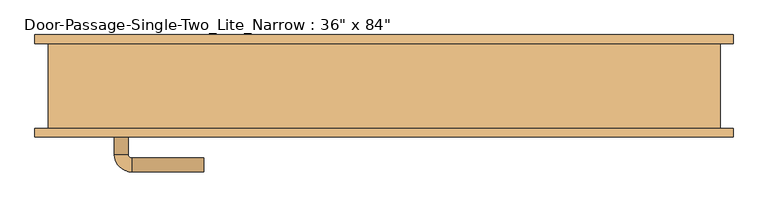
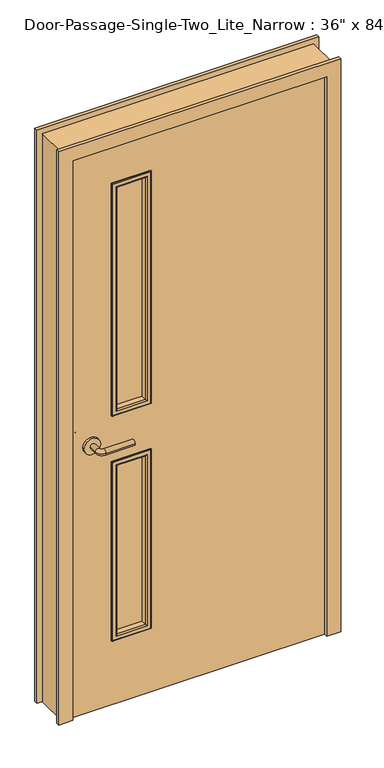
"""IFC4 building model written with IfcOpenShell, lengths in millimetres: door geometry."""

from ifc_helpers import new_model, si_unit, point, frame, frame_2d, origin, place, context, project, spatial, polyline, circle_curve, ellipse_curve, trimmed, segment, composite_curve, outline, extrude, faceted_brep, source, transform, mapped, element, save
from ifc_brep_helpers import plane_surface, cylinder_surface, revolved_surface, advanced_brep


def door_7eef6684(model_context):
    return source(origin(), model_context, "Body", "SolidModel", [
        advanced_brep(
        [(-392.190625, -15.8125, 1016.0), (-372.190625, -15.8125, 1016.0), (-392.190625, 14.1875, 1016.0), (-372.190625, 14.1875, 1016.0), (-367.190625, 19.1875, 1016.0), (-367.190625, 39.1875, 1016.0), (-262.190625, 39.1875, 1016.0), (-262.190625, 19.1875, 1016.0)],
        [
            (0, 1, circle_curve(frame((-382.190625, -15.8125, 1016.0), z_axis=(0.0, -1.0, 0.0), x_axis=(1.0, 0.0, 0.0)), 10.0)),
            (1, 0, circle_curve(frame((-382.190625, -15.8125, 1016.0), z_axis=(0.0, -1.0, 0.0), x_axis=(1.0, 0.0, 0.0)), 10.0)),
            (0, 2),
            (2, 3, circle_curve(frame((-382.190625, 14.1875, 1016.0), z_axis=(0.0, -1.0, 0.0), x_axis=(1.0, 0.0, 0.0)), 10.0)),
            (3, 1),
            (3, 2, circle_curve(frame((-382.190625, 14.1875, 1016.0), z_axis=(0.0, -1.0, 0.0), x_axis=(1.0, 0.0, 0.0)), 10.0)),
            (4, 3, circle_curve(frame((-367.190625, 14.1875, 1016.0), z_axis=(0.0, 0.0, 1.0), x_axis=(-1.0, 0.0, 0.0)), 5.0)),
            (2, 5, circle_curve(frame((-367.190625, 14.1875, 1016.0), z_axis=(0.0, 0.0, -1.0), x_axis=(-1.0, 0.0, 0.0)), 25.0)),
            (5, 4, circle_curve(frame((-367.190625, 29.1875, 1016.0), z_axis=(-1.0, 0.0, 0.0), x_axis=(0.0, -1.0, 0.0)), 10.0)),
            (4, 5, circle_curve(frame((-367.190625, 29.1875, 1016.0), z_axis=(-1.0, 0.0, 0.0), x_axis=(0.0, -1.0, 0.0)), 10.0)),
            (6, 7, circle_curve(frame((-262.190625, 29.1875, 1016.0), z_axis=(1.0, 0.0, 0.0), x_axis=(0.0, -1.0, 0.0)), 10.0)),
            (7, 6, circle_curve(frame((-262.190625, 29.1875, 1016.0), z_axis=(1.0, 0.0, 0.0), x_axis=(0.0, -1.0, 0.0)), 10.0)),
            (5, 6),
            (7, 4),
        ],
        [
            plane_surface(frame((-382.190625, -15.8125, 1016.0), z_axis=(0.0, -1.0, 0.0), x_axis=(0.0, 0.0, 1.0))),
            cylinder_surface(frame((-382.190625, -15.8125, 1016.0), z_axis=(0.0, -1.0, 0.0), x_axis=(1.0, 0.0, 0.0)), 10.0),
            revolved_surface(trimmed(ellipse_curve(frame((-382.190625, 14.1875, 1016.0), z_axis=(0.0, -1.0, 0.0), x_axis=(1.0, 0.0, 0.0)), 10.0, 10.0), [point((-392.190625, 14.1875, 1016.0))], [point((-372.190625, 14.1875, 1016.0))], True, "CARTESIAN"), (-367.190625, 14.1875, 1016.0), (0.0, 0.0, -1.0)),
            revolved_surface(trimmed(ellipse_curve(frame((-382.190625, 14.1875, 1016.0), z_axis=(0.0, -1.0, 0.0), x_axis=(1.0, 0.0, 0.0)), 10.0, 10.0), [point((-372.190625, 14.1875, 1016.0))], [point((-392.190625, 14.1875, 1016.0))], True, "CARTESIAN"), (-367.190625, 14.1875, 1016.0), (0.0, 0.0, -1.0)),
            plane_surface(frame((-262.190625, 29.1875, 1016.0), z_axis=(1.0, 0.0, 0.0), x_axis=(0.0, 0.0, 1.0))),
            cylinder_surface(frame((-367.190625, 29.1875, 1016.0), z_axis=(-1.0, 0.0, 0.0), x_axis=(0.0, -1.0, 0.0)), 10.0),
        ],
        [
            (0, [[1, 2]]),
            (1, [[-1, 3, 4, 5]]),
            (1, [[-2, -5, 6, -3]]),
            (2, [[7, -4, 8, 9]]),
            (3, [[-8, -6, -7, 10]]),
            (4, [[11, 12]]),
            (5, [[-9, 13, -12, 14]]),
            (5, [[-10, -14, -11, -13]]),
        ],
    ),
        extrude(outline(composite_curve([segment(trimmed(circle_curve(frame_2d((1016.0, -384.690625)), 30.0), [point((1016.0, -414.690625))], [point((1016.0, -354.690625))], False, "CARTESIAN"), True, "CONTINUOUS"), segment(trimmed(circle_curve(frame_2d((1016.0, -384.690625)), 30.0), [point((1016.0, -354.690625))], [point((1016.0, -414.690625))], False, "CARTESIAN"), True, "CONTINUOUS")], self_intersect=False)), frame((0.0, -23.8125, 0.0), z_axis=(0.0, 1.0, 0.0), x_axis=(0.0, 0.0, 1.0)), (0.0, 0.0, 1.0), 8.0),
        advanced_brep(
        [(-392.190625, -76.2625, 1016.0), (-372.190625, -76.2625, 1016.0), (-372.190625, -106.2625, 1016.0), (-392.190625, -106.2625, 1016.0), (-367.190625, -111.2625, 1016.0), (-367.190625, -131.2625, 1016.0), (-262.190625, -131.2625, 1016.0), (-262.190625, -111.2625, 1016.0)],
        [
            (0, 1, circle_curve(frame((-382.190625, -76.2625, 1016.0), z_axis=(0.0, 1.0, 0.0), x_axis=(1.0, 0.0, 0.0)), 10.0)),
            (1, 0, circle_curve(frame((-382.190625, -76.2625, 1016.0), z_axis=(0.0, 1.0, 0.0), x_axis=(1.0, 0.0, 0.0)), 10.0)),
            (1, 2),
            (2, 3, circle_curve(frame((-382.190625, -106.2625, 1016.0), z_axis=(0.0, 1.0, 0.0), x_axis=(1.0, 0.0, 0.0)), 10.0)),
            (3, 0),
            (3, 2, circle_curve(frame((-382.190625, -106.2625, 1016.0), z_axis=(0.0, 1.0, 0.0), x_axis=(1.0, 0.0, 0.0)), 10.0)),
            (4, 5, circle_curve(frame((-367.190625, -121.2625, 1016.0), z_axis=(-1.0, 0.0, 0.0), x_axis=(0.0, 1.0, 0.0)), 10.0)),
            (5, 3, circle_curve(frame((-367.190625, -106.2625, 1016.0), z_axis=(0.0, 0.0, -1.0), x_axis=(-1.0, 0.0, 0.0)), 25.0)),
            (2, 4, circle_curve(frame((-367.190625, -106.2625, 1016.0), z_axis=(0.0, 0.0, 1.0), x_axis=(-1.0, 0.0, 0.0)), 5.0)),
            (5, 4, circle_curve(frame((-367.190625, -121.2625, 1016.0), z_axis=(-1.0, 0.0, 0.0), x_axis=(0.0, 1.0, 0.0)), 10.0)),
            (6, 7, circle_curve(frame((-262.190625, -121.2625, 1016.0), z_axis=(1.0, 0.0, 0.0), x_axis=(0.0, 1.0, 0.0)), 10.0)),
            (7, 6, circle_curve(frame((-262.190625, -121.2625, 1016.0), z_axis=(1.0, 0.0, 0.0), x_axis=(0.0, 1.0, 0.0)), 10.0)),
            (4, 7),
            (6, 5),
        ],
        [
            plane_surface(frame((-382.190625, -76.2625, 1016.0), z_axis=(0.0, 1.0, 0.0), x_axis=(0.0, 0.0, 1.0))),
            cylinder_surface(frame((-382.190625, -76.2625, 1016.0), z_axis=(0.0, 1.0, 0.0), x_axis=(1.0, 0.0, 0.0)), 10.0),
            revolved_surface(trimmed(ellipse_curve(frame((-382.190625, -106.2625, 1016.0), z_axis=(0.0, -1.0, 0.0), x_axis=(1.0, 0.0, 0.0)), 10.0, 10.0), [point((-392.190625, -106.2625, 1016.0))], [point((-372.190625, -106.2625, 1016.0))], True, "CARTESIAN"), (-367.190625, -106.2625, 1016.0), (0.0, 0.0, -1.0)),
            revolved_surface(trimmed(ellipse_curve(frame((-382.190625, -106.2625, 1016.0), z_axis=(0.0, -1.0, 0.0), x_axis=(1.0, 0.0, 0.0)), 10.0, 10.0), [point((-372.190625, -106.2625, 1016.0))], [point((-392.190625, -106.2625, 1016.0))], True, "CARTESIAN"), (-367.190625, -106.2625, 1016.0), (0.0, 0.0, -1.0)),
            plane_surface(frame((-262.190625, -121.2625, 1016.0), z_axis=(1.0, 0.0, 0.0), x_axis=(0.0, 0.0, 1.0))),
            cylinder_surface(frame((-367.190625, -121.2625, 1016.0), z_axis=(-1.0, 0.0, 0.0), x_axis=(0.0, 1.0, 0.0)), 10.0),
        ],
        [
            (0, [[1, 2]]),
            (1, [[3, 4, 5, -2]]),
            (1, [[-5, 6, -3, -1]]),
            (2, [[7, 8, -4, 9]]),
            (3, [[10, -9, -6, -8]]),
            (4, [[11, 12]]),
            (5, [[13, -11, 14, -7]]),
            (5, [[-14, -12, -13, -10]]),
        ],
    ),
        extrude(outline(composite_curve([segment(trimmed(circle_curve(frame_2d((1016.0, -384.690625)), 30.0), [point((1016.0, -414.690625))], [point((1016.0, -354.690625))], False, "CARTESIAN"), True, "CONTINUOUS"), segment(trimmed(circle_curve(frame_2d((1016.0, -384.690625)), 30.0), [point((1016.0, -354.690625))], [point((1016.0, -414.690625))], False, "CARTESIAN"), True, "CONTINUOUS")], self_intersect=False)), frame((0.0, -76.2625, 0.0), z_axis=(0.0, 1.0, 0.0), x_axis=(0.0, 0.0, 1.0)), (0.0, 0.0, 1.0), 8.0),
        faceted_brep([(457.2, -80.9625, 0.0), (457.2, -19.05, 0.0), (441.325, -19.05, 0.0), (441.325, 19.05, 0.0), (457.2, 19.05, 0.0), (457.2, 68.2625, 0.0), (508.0, 68.2625, 0.0), (508.0, 55.5625, 0.0), (488.95, 55.5625, 0.0), (488.95, -68.2625, 0.0), (508.0, -68.2625, 0.0), (508.0, -80.9625, 0.0), (508.0, -80.9625, 2184.4), (-508.0, -80.9625, 2184.4), (-508.0, -80.9625, 0.0), (-457.2, -80.9625, 0.0), (-457.2, -80.9625, 2133.6), (457.2, -80.9625, 2133.6), (508.0, -68.2625, 2184.4), (488.95, -68.2625, 2165.35), (-488.95, -68.2625, 2165.35), (-488.95, -68.2625, 0.0), (-508.0, -68.2625, 0.0), (-508.0, -68.2625, 2184.4), (488.95, 55.5625, 2165.35), (508.0, 55.5625, 2184.4), (-508.0, 55.5625, 2184.4), (-508.0, 55.5625, 0.0), (-488.95, 55.5625, 0.0), (-488.95, 55.5625, 2165.35), (508.0, 68.2625, 2184.4), (457.2, 68.2625, 2133.6), (-457.2, 68.2625, 2133.6), (-457.2, 68.2625, 0.0), (-508.0, 68.2625, 0.0), (-508.0, 68.2625, 2184.4), (457.2, 19.05, 2133.6), (441.325, 19.05, 2117.725), (-441.325, 19.05, 2117.725), (-441.325, 19.05, 0.0), (-457.2, 19.05, 0.0), (-457.2, 19.05, 2133.6), (441.325, -19.05, 2117.725), (457.2, -19.05, 2133.6), (-457.2, -19.05, 2133.6), (-457.2, -19.05, 0.0), (-441.325, -19.05, 0.0), (-441.325, -19.05, 2117.725)], [[[0, 1, 2, 3, 4, 5, 6, 7, 8, 9, 10, 11]], [[11, 12, 13, 14, 15, 16, 17, 0]], [[10, 18, 12, 11]], [[9, 19, 20, 21, 22, 23, 18, 10]], [[8, 24, 19, 9]], [[7, 25, 26, 27, 28, 29, 24, 8]], [[6, 30, 25, 7]], [[5, 31, 32, 33, 34, 35, 30, 6]], [[4, 36, 31, 5]], [[3, 37, 38, 39, 40, 41, 36, 4]], [[2, 42, 37, 3]], [[1, 43, 44, 45, 46, 47, 42, 2]], [[0, 17, 43, 1]], [[18, 23, 13, 12]], [[24, 29, 20, 19]], [[30, 35, 26, 25]], [[36, 41, 32, 31]], [[42, 47, 38, 37]], [[17, 16, 44, 43]], [[15, 14, 22, 21, 28, 27, 34, 33, 40, 39, 46, 45]], [[23, 22, 14, 13]], [[29, 28, 21, 20]], [[35, 34, 27, 26]], [[41, 40, 33, 32]], [[47, 46, 39, 38]], [[16, 15, 45, 44]]]),
        extrude(outline(polyline([(2133.6, -457.2), (0.0, -457.2), (0.0, 457.2), (2133.6, 457.2), (2133.6, -457.2)]), holes=[polyline([(1981.2, -304.8), (1981.2, -177.8), (1111.25, -177.8), (1111.25, -304.8), (1981.2, -304.8)]), polyline([(920.75, -304.8), (920.75, -177.8), (254.0, -177.8), (254.0, -304.8), (920.75, -304.8)])]), frame((0.0, -68.2625, 0.0), z_axis=(0.0, 1.0, 0.0), x_axis=(0.0, 0.0, 1.0)), (0.0, 0.0, 1.0), 44.45),
        extrude(outline(polyline([(-177.8, -42.8625), (-177.8, -49.2125), (-304.8, -49.2125), (-304.8, -42.8625), (-177.8, -42.8625)])), frame((0.0, 0.0, 1111.25), z_axis=(0.0, 0.0, 1.0), x_axis=(1.0, 0.0, 0.0)), (0.0, 0.0, 1.0), 869.95),
        extrude(outline(polyline([(-177.8, -42.8625), (-177.8, -49.2125), (-304.8, -49.2125), (-304.8, -42.8625), (-177.8, -42.8625)])), frame((0.0, 0.0, 254.0), z_axis=(0.0, 0.0, 1.0), x_axis=(1.0, 0.0, 0.0)), (0.0, 0.0, 1.0), 666.75),
        advanced_brep(
        [(-177.8, -42.8625, 920.75), (-177.8, -42.8625, 254.0), (-177.8, -23.8125, 254.0), (-177.8, -23.8125, 920.75), (-189.8, -22.8125, 908.75), (-189.8, -22.8125, 266.0), (-189.8, -42.8625, 266.0), (-189.8, -42.8625, 908.75), (-184.8, -17.8125, 913.75), (-184.8, -17.8125, 261.0), (-169.8, -19.8125, 928.75), (-169.8, -19.8125, 246.0), (-171.8, -17.8125, 248.0), (-171.8, -17.8125, 926.75), (-169.8, -23.8125, 928.75), (-169.8, -23.8125, 246.0), (-304.8, -42.8625, 254.0), (-304.8, -23.8125, 254.0), (-292.8, -22.8125, 266.0), (-292.8, -42.8625, 266.0), (-297.8, -17.8125, 261.0), (-312.8, -19.8125, 246.0), (-310.8, -17.8125, 248.0), (-312.8, -23.8125, 246.0), (-304.8, -42.8625, 920.75), (-304.8, -23.8125, 920.75), (-292.8, -22.8125, 908.75), (-292.8, -42.8625, 908.75), (-297.8, -17.8125, 913.75), (-312.8, -19.8125, 928.75), (-310.8, -17.8125, 926.75), (-312.8, -23.8125, 928.75)],
        [
            (0, 1),
            (1, 2),
            (2, 3),
            (3, 0),
            (4, 5),
            (5, 6),
            (6, 7),
            (7, 4),
            (8, 9),
            (9, 5, ellipse_curve(frame((-184.8, -22.8125, 261.0), z_axis=(0.7071067811865475, 0.0, 0.7071067811865475), x_axis=(-0.7071067811865474, 0.0, 0.7071067811865476)), 7.0710678, 5.0)),
            (4, 8, ellipse_curve(frame((-184.8, -22.8125, 913.75), z_axis=(0.7071067811865475, 0.0, -0.7071067811865475), x_axis=(0.7071067811865474, 0.0, 0.7071067811865476)), 7.0710678, 5.0)),
            (10, 11),
            (11, 12, ellipse_curve(frame((-171.8, -19.8125, 248.0), z_axis=(0.7071067811865475, 0.0, 0.7071067811865475), x_axis=(-0.7071067811865474, 0.0, 0.7071067811865476)), 2.8284271, 2.0)),
            (12, 13),
            (13, 10, ellipse_curve(frame((-171.8, -19.8125, 926.75), z_axis=(0.7071067811865475, 0.0, -0.7071067811865475), x_axis=(0.7071067811865474, 0.0, 0.7071067811865476)), 2.8284271, 2.0)),
            (14, 15),
            (15, 11),
            (10, 14),
            (1, 16),
            (16, 17),
            (17, 2),
            (5, 18),
            (18, 19),
            (19, 6),
            (9, 20),
            (20, 18, ellipse_curve(frame((-297.8, -22.8125, 261.0), z_axis=(0.7071067811865475, 0.0, -0.7071067811865475), x_axis=(0.7071067811865476, 0.0, 0.7071067811865474)), 7.0710678, 5.0)),
            (11, 21),
            (21, 22, ellipse_curve(frame((-310.8, -19.8125, 248.0), z_axis=(0.7071067811865475, 0.0, -0.7071067811865475), x_axis=(0.7071067811865476, 0.0, 0.7071067811865474)), 2.8284271, 2.0)),
            (22, 12),
            (15, 23),
            (23, 21),
            (16, 24),
            (24, 25),
            (25, 17),
            (18, 26),
            (26, 27),
            (27, 19),
            (20, 28),
            (28, 26, ellipse_curve(frame((-297.8, -22.8125, 913.75), z_axis=(-0.7071067811865475, 0.0, -0.7071067811865475), x_axis=(0.7071067811865474, 0.0, -0.7071067811865476)), 7.0710678, 5.0)),
            (21, 29),
            (29, 30, ellipse_curve(frame((-310.8, -19.8125, 926.75), z_axis=(-0.7071067811865475, 0.0, -0.7071067811865475), x_axis=(0.7071067811865474, 0.0, -0.7071067811865476)), 2.8284271, 2.0)),
            (30, 22),
            (23, 31),
            (31, 29),
            (14, 31),
            (25, 3),
            (24, 0),
            (27, 7),
            (26, 4),
            (28, 8),
            (30, 13),
            (29, 10),
        ],
        [
            plane_surface(frame((-177.8, -23.8125, 920.75), z_axis=(1.0, 0.0, 0.0), x_axis=(0.0, 0.0, -1.0))),
            plane_surface(frame((-189.8, -42.8625, 908.75), z_axis=(-1.0, 0.0, 0.0), x_axis=(0.0, 0.0, -1.0))),
            cylinder_surface(frame((-184.8, -22.8125, 920.75), z_axis=(0.0, 0.0, 1.0), x_axis=(1.0, 0.0, 0.0)), 5.0),
            cylinder_surface(frame((-171.8, -19.8125, 920.75), z_axis=(0.0, 0.0, 1.0), x_axis=(1.0, 0.0, 0.0)), 2.0),
            plane_surface(frame((-169.8, -19.8125, 928.75), z_axis=(1.0, 0.0, 0.0), x_axis=(0.0, 0.0, -1.0))),
            plane_surface(frame((-177.8, -23.8125, 254.0), z_axis=(0.0, 0.0, -1.0), x_axis=(-1.0, 0.0, 0.0))),
            plane_surface(frame((-189.8, -42.8625, 266.0), z_axis=(0.0, 0.0, 1.0), x_axis=(-1.0, 0.0, 0.0))),
            cylinder_surface(frame((-177.8, -22.8125, 261.0), z_axis=(1.0, 0.0, 0.0), x_axis=(0.0, 0.0, -1.0)), 5.0),
            cylinder_surface(frame((-177.8, -19.8125, 248.0), z_axis=(1.0, 0.0, 0.0), x_axis=(0.0, 0.0, -1.0)), 2.0),
            plane_surface(frame((-169.8, -19.8125, 246.0), z_axis=(0.0, 0.0, -1.0), x_axis=(-1.0, 0.0, 0.0))),
            plane_surface(frame((-304.8, -23.8125, 254.0), z_axis=(-1.0, 0.0, 0.0), x_axis=(0.0, 0.0, 1.0))),
            plane_surface(frame((-292.8, -42.8625, 266.0), z_axis=(1.0, 0.0, 0.0), x_axis=(0.0, 0.0, 1.0))),
            cylinder_surface(frame((-297.8, -22.8125, 254.0), z_axis=(0.0, 0.0, -1.0), x_axis=(-1.0, 0.0, 0.0)), 5.0),
            cylinder_surface(frame((-310.8, -19.8125, 254.0), z_axis=(0.0, 0.0, -1.0), x_axis=(-1.0, 0.0, 0.0)), 2.0),
            plane_surface(frame((-312.8, -19.8125, 246.0), z_axis=(-1.0, 0.0, 0.0), x_axis=(0.0, 0.0, 1.0))),
            plane_surface(frame((-312.8, -23.8125, 928.75), z_axis=(0.0, -1.0, 0.0), x_axis=(1.0, 0.0, 0.0))),
            plane_surface(frame((-304.8, -23.8125, 920.75), z_axis=(0.0, 0.0, 1.0), x_axis=(1.0, 0.0, 0.0))),
            plane_surface(frame((-304.8, -42.8625, 920.75), z_axis=(0.0, -1.0, 0.0), x_axis=(1.0, 0.0, 0.0))),
            plane_surface(frame((-292.8, -42.8625, 908.75), z_axis=(0.0, 0.0, -1.0), x_axis=(1.0, 0.0, 0.0))),
            cylinder_surface(frame((-304.8, -22.8125, 913.75), z_axis=(-1.0, 0.0, 0.0), x_axis=(0.0, 0.0, 1.0)), 5.0),
            plane_surface(frame((-297.8, -17.8125, 913.75), z_axis=(0.0, 1.0, 0.0), x_axis=(1.0, 0.0, 0.0))),
            cylinder_surface(frame((-304.8, -19.8125, 926.75), z_axis=(-1.0, 0.0, 0.0), x_axis=(0.0, 0.0, 1.0)), 2.0),
            plane_surface(frame((-312.8, -19.8125, 928.75), z_axis=(0.0, 0.0, 1.0), x_axis=(1.0, 0.0, 0.0))),
        ],
        [
            (0, [[1, 2, 3, 4]]),
            (1, [[5, 6, 7, 8]]),
            (2, [[9, 10, -5, 11]]),
            (3, [[12, 13, 14, 15]]),
            (4, [[16, 17, -12, 18]]),
            (5, [[19, 20, 21, -2]]),
            (6, [[22, 23, 24, -6]]),
            (7, [[25, 26, -22, -10]]),
            (8, [[27, 28, 29, -13]]),
            (9, [[30, 31, -27, -17]]),
            (10, [[32, 33, 34, -20]]),
            (11, [[35, 36, 37, -23]]),
            (12, [[38, 39, -35, -26]]),
            (13, [[40, 41, 42, -28]]),
            (14, [[43, 44, -40, -31]]),
            (15, [[-16, 45, -43, -30], [-3, -21, -34, 46]]),
            (16, [[47, -4, -46, -33]]),
            (17, [[-1, -47, -32, -19], [-7, -24, -37, 48]]),
            (18, [[49, -8, -48, -36]]),
            (19, [[50, -11, -49, -39]]),
            (20, [[-14, -29, -42, 51], [-9, -50, -38, -25]]),
            (21, [[52, -15, -51, -41]]),
            (22, [[-45, -18, -52, -44]]),
        ],
    ),
        advanced_brep(
        [(-304.8, -49.2125, 920.75), (-304.8, -49.2125, 254.0), (-304.8, -68.2625, 254.0), (-304.8, -68.2625, 920.75), (-292.8, -69.2625, 908.75), (-292.8, -69.2625, 266.0), (-292.8, -49.2125, 266.0), (-292.8, -49.2125, 908.75), (-297.8, -74.2625, 913.75), (-297.8, -74.2625, 261.0), (-312.8, -72.2625, 928.75), (-312.8, -72.2625, 246.0), (-310.8, -74.2625, 248.0), (-310.8, -74.2625, 926.75), (-312.8, -68.2625, 928.75), (-312.8, -68.2625, 246.0), (-177.8, -49.2125, 254.0), (-177.8, -68.2625, 254.0), (-189.8, -69.2625, 266.0), (-189.8, -49.2125, 266.0), (-184.8, -74.2625, 261.0), (-169.8, -72.2625, 246.0), (-171.8, -74.2625, 248.0), (-169.8, -68.2625, 246.0), (-177.8, -49.2125, 920.75), (-177.8, -68.2625, 920.75), (-189.8, -69.2625, 908.75), (-189.8, -49.2125, 908.75), (-184.8, -74.2625, 913.75), (-169.8, -72.2625, 928.75), (-171.8, -74.2625, 926.75), (-169.8, -68.2625, 928.75)],
        [
            (0, 1),
            (1, 2),
            (2, 3),
            (3, 0),
            (4, 5),
            (5, 6),
            (6, 7),
            (7, 4),
            (8, 9),
            (9, 5, ellipse_curve(frame((-297.8, -69.2625, 261.0), z_axis=(-0.7071067811865475, 0.0, 0.7071067811865475), x_axis=(0.7071067811865474, 0.0, 0.7071067811865476)), 7.0710678, 5.0)),
            (4, 8, ellipse_curve(frame((-297.8, -69.2625, 913.75), z_axis=(-0.7071067811865475, 0.0, -0.7071067811865475), x_axis=(-0.7071067811865474, 0.0, 0.7071067811865476)), 7.0710678, 5.0)),
            (10, 11),
            (11, 12, ellipse_curve(frame((-310.8, -72.2625, 248.0), z_axis=(-0.7071067811865475, 0.0, 0.7071067811865475), x_axis=(0.7071067811865474, 0.0, 0.7071067811865476)), 2.8284271, 2.0)),
            (12, 13),
            (13, 10, ellipse_curve(frame((-310.8, -72.2625, 926.75), z_axis=(-0.7071067811865475, 0.0, -0.7071067811865475), x_axis=(-0.7071067811865474, 0.0, 0.7071067811865476)), 2.8284271, 2.0)),
            (14, 15),
            (15, 11),
            (10, 14),
            (1, 16),
            (16, 17),
            (17, 2),
            (5, 18),
            (18, 19),
            (19, 6),
            (9, 20),
            (20, 18, ellipse_curve(frame((-184.8, -69.2625, 261.0), z_axis=(-0.7071067811865475, 0.0, -0.7071067811865475), x_axis=(-0.7071067811865476, 0.0, 0.7071067811865474)), 7.0710678, 5.0)),
            (11, 21),
            (21, 22, ellipse_curve(frame((-171.8, -72.2625, 248.0), z_axis=(-0.7071067811865475, 0.0, -0.7071067811865475), x_axis=(-0.7071067811865476, 0.0, 0.7071067811865474)), 2.8284271, 2.0)),
            (22, 12),
            (15, 23),
            (23, 21),
            (16, 24),
            (24, 25),
            (25, 17),
            (18, 26),
            (26, 27),
            (27, 19),
            (20, 28),
            (28, 26, ellipse_curve(frame((-184.8, -69.2625, 913.75), z_axis=(0.7071067811865475, 0.0, -0.7071067811865475), x_axis=(-0.7071067811865474, 0.0, -0.7071067811865476)), 7.0710678, 5.0)),
            (21, 29),
            (29, 30, ellipse_curve(frame((-171.8, -72.2625, 926.75), z_axis=(0.7071067811865475, 0.0, -0.7071067811865475), x_axis=(-0.7071067811865474, 0.0, -0.7071067811865476)), 2.8284271, 2.0)),
            (30, 22),
            (23, 31),
            (31, 29),
            (14, 31),
            (25, 3),
            (24, 0),
            (27, 7),
            (26, 4),
            (28, 8),
            (30, 13),
            (29, 10),
        ],
        [
            plane_surface(frame((-304.8, -68.2625, 920.75), z_axis=(-1.0, 0.0, 0.0), x_axis=(0.0, 0.0, -1.0))),
            plane_surface(frame((-292.8, -49.2125, 908.75), z_axis=(1.0, 0.0, 0.0), x_axis=(0.0, 0.0, -1.0))),
            cylinder_surface(frame((-297.8, -69.2625, 920.75), z_axis=(0.0, 0.0, 1.0), x_axis=(-1.0, 0.0, 0.0)), 5.0),
            cylinder_surface(frame((-310.8, -72.2625, 920.75), z_axis=(0.0, 0.0, 1.0), x_axis=(-1.0, 0.0, 0.0)), 2.0),
            plane_surface(frame((-312.8, -72.2625, 928.75), z_axis=(-1.0, 0.0, 0.0), x_axis=(0.0, 0.0, -1.0))),
            plane_surface(frame((-304.8, -68.2625, 254.0), z_axis=(0.0, 0.0, -1.0), x_axis=(1.0, 0.0, 0.0))),
            plane_surface(frame((-292.8, -49.2125, 266.0), z_axis=(0.0, 0.0, 1.0), x_axis=(1.0, 0.0, 0.0))),
            cylinder_surface(frame((-304.8, -69.2625, 261.0), z_axis=(-1.0, 0.0, 0.0), x_axis=(0.0, 0.0, -1.0)), 5.0),
            cylinder_surface(frame((-304.8, -72.2625, 248.0), z_axis=(-1.0, 0.0, 0.0), x_axis=(0.0, 0.0, -1.0)), 2.0),
            plane_surface(frame((-312.8, -72.2625, 246.0), z_axis=(0.0, 0.0, -1.0), x_axis=(1.0, 0.0, 0.0))),
            plane_surface(frame((-177.8, -68.2625, 254.0), z_axis=(1.0, 0.0, 0.0), x_axis=(0.0, 0.0, 1.0))),
            plane_surface(frame((-189.8, -49.2125, 266.0), z_axis=(-1.0, 0.0, 0.0), x_axis=(0.0, 0.0, 1.0))),
            cylinder_surface(frame((-184.8, -69.2625, 254.0), z_axis=(0.0, 0.0, -1.0), x_axis=(1.0, 0.0, 0.0)), 5.0),
            cylinder_surface(frame((-171.8, -72.2625, 254.0), z_axis=(0.0, 0.0, -1.0), x_axis=(1.0, 0.0, 0.0)), 2.0),
            plane_surface(frame((-169.8, -72.2625, 246.0), z_axis=(1.0, 0.0, 0.0), x_axis=(0.0, 0.0, 1.0))),
            plane_surface(frame((-169.8, -68.2625, 928.75), z_axis=(0.0, 1.0, 0.0), x_axis=(-1.0, 0.0, 0.0))),
            plane_surface(frame((-177.8, -68.2625, 920.75), z_axis=(0.0, 0.0, 1.0), x_axis=(-1.0, 0.0, 0.0))),
            plane_surface(frame((-177.8, -49.2125, 920.75), z_axis=(0.0, 1.0, 0.0), x_axis=(-1.0, 0.0, 0.0))),
            plane_surface(frame((-189.8, -49.2125, 908.75), z_axis=(0.0, 0.0, -1.0), x_axis=(-1.0, 0.0, 0.0))),
            cylinder_surface(frame((-177.8, -69.2625, 913.75), z_axis=(1.0, 0.0, 0.0), x_axis=(0.0, 0.0, 1.0)), 5.0),
            plane_surface(frame((-184.8, -74.2625, 913.75), z_axis=(0.0, -1.0, 0.0), x_axis=(-1.0, 0.0, 0.0))),
            cylinder_surface(frame((-177.8, -72.2625, 926.75), z_axis=(1.0, 0.0, 0.0), x_axis=(0.0, 0.0, 1.0)), 2.0),
            plane_surface(frame((-169.8, -72.2625, 928.75), z_axis=(0.0, 0.0, 1.0), x_axis=(-1.0, 0.0, 0.0))),
        ],
        [
            (0, [[1, 2, 3, 4]]),
            (1, [[5, 6, 7, 8]]),
            (2, [[9, 10, -5, 11]]),
            (3, [[12, 13, 14, 15]]),
            (4, [[16, 17, -12, 18]]),
            (5, [[19, 20, 21, -2]]),
            (6, [[22, 23, 24, -6]]),
            (7, [[25, 26, -22, -10]]),
            (8, [[27, 28, 29, -13]]),
            (9, [[30, 31, -27, -17]]),
            (10, [[32, 33, 34, -20]]),
            (11, [[35, 36, 37, -23]]),
            (12, [[38, 39, -35, -26]]),
            (13, [[40, 41, 42, -28]]),
            (14, [[43, 44, -40, -31]]),
            (15, [[-16, 45, -43, -30], [-3, -21, -34, 46]]),
            (16, [[47, -4, -46, -33]]),
            (17, [[-1, -47, -32, -19], [-7, -24, -37, 48]]),
            (18, [[49, -8, -48, -36]]),
            (19, [[50, -11, -49, -39]]),
            (20, [[-14, -29, -42, 51], [-9, -50, -38, -25]]),
            (21, [[52, -15, -51, -41]]),
            (22, [[-45, -18, -52, -44]]),
        ],
    ),
        advanced_brep(
        [(-304.8, -42.8625, 1111.25), (-304.8, -42.8625, 1981.2), (-304.8, -23.8125, 1981.2), (-304.8, -23.8125, 1111.25), (-292.8, -22.8125, 1123.25), (-292.8, -22.8125, 1969.2), (-292.8, -42.8625, 1969.2), (-292.8, -42.8625, 1123.25), (-297.8, -17.8125, 1118.25), (-297.8, -17.8125, 1974.2), (-312.8, -19.8125, 1103.25), (-312.8, -19.8125, 1989.2), (-310.8, -17.8125, 1987.2), (-310.8, -17.8125, 1105.25), (-312.8, -23.8125, 1103.25), (-312.8, -23.8125, 1989.2), (-177.8, -42.8625, 1981.2), (-177.8, -23.8125, 1981.2), (-189.8, -22.8125, 1969.2), (-189.8, -42.8625, 1969.2), (-184.8, -17.8125, 1974.2), (-169.8, -19.8125, 1989.2), (-171.8, -17.8125, 1987.2), (-169.8, -23.8125, 1989.2), (-177.8, -42.8625, 1111.25), (-177.8, -23.8125, 1111.25), (-189.8, -22.8125, 1123.25), (-189.8, -42.8625, 1123.25), (-184.8, -17.8125, 1118.25), (-169.8, -19.8125, 1103.25), (-171.8, -17.8125, 1105.25), (-169.8, -23.8125, 1103.25)],
        [
            (0, 1),
            (1, 2),
            (2, 3),
            (3, 0),
            (4, 5),
            (5, 6),
            (6, 7),
            (7, 4),
            (8, 9),
            (9, 5, ellipse_curve(frame((-297.8, -22.8125, 1974.2), z_axis=(-0.7071067811865475, 0.0, -0.7071067811865475), x_axis=(0.7071067811865474, 0.0, -0.7071067811865476)), 7.0710678, 5.0)),
            (4, 8, ellipse_curve(frame((-297.8, -22.8125, 1118.25), z_axis=(-0.7071067811865475, 0.0, 0.7071067811865475), x_axis=(-0.7071067811865474, 0.0, -0.7071067811865476)), 7.0710678, 5.0)),
            (10, 11),
            (11, 12, ellipse_curve(frame((-310.8, -19.8125, 1987.2), z_axis=(-0.7071067811865475, 0.0, -0.7071067811865475), x_axis=(0.7071067811865474, 0.0, -0.7071067811865476)), 2.8284271, 2.0)),
            (12, 13),
            (13, 10, ellipse_curve(frame((-310.8, -19.8125, 1105.25), z_axis=(-0.7071067811865475, 0.0, 0.7071067811865475), x_axis=(-0.7071067811865474, 0.0, -0.7071067811865476)), 2.8284271, 2.0)),
            (14, 15),
            (15, 11),
            (10, 14),
            (1, 16),
            (16, 17),
            (17, 2),
            (5, 18),
            (18, 19),
            (19, 6),
            (9, 20),
            (20, 18, ellipse_curve(frame((-184.8, -22.8125, 1974.2), z_axis=(-0.7071067811865475, 0.0, 0.7071067811865475), x_axis=(-0.7071067811865476, 0.0, -0.7071067811865474)), 7.0710678, 5.0)),
            (11, 21),
            (21, 22, ellipse_curve(frame((-171.8, -19.8125, 1987.2), z_axis=(-0.7071067811865475, 0.0, 0.7071067811865475), x_axis=(-0.7071067811865476, 0.0, -0.7071067811865474)), 2.8284271, 2.0)),
            (22, 12),
            (15, 23),
            (23, 21),
            (16, 24),
            (24, 25),
            (25, 17),
            (18, 26),
            (26, 27),
            (27, 19),
            (20, 28),
            (28, 26, ellipse_curve(frame((-184.8, -22.8125, 1118.25), z_axis=(0.7071067811865475, 0.0, 0.7071067811865475), x_axis=(-0.7071067811865474, 0.0, 0.7071067811865476)), 7.0710678, 5.0)),
            (21, 29),
            (29, 30, ellipse_curve(frame((-171.8, -19.8125, 1105.25), z_axis=(0.7071067811865475, 0.0, 0.7071067811865475), x_axis=(-0.7071067811865474, 0.0, 0.7071067811865476)), 2.8284271, 2.0)),
            (30, 22),
            (23, 31),
            (31, 29),
            (14, 31),
            (25, 3),
            (24, 0),
            (27, 7),
            (26, 4),
            (28, 8),
            (30, 13),
            (29, 10),
        ],
        [
            plane_surface(frame((-304.8, -23.8125, 1111.25), z_axis=(-1.0, 0.0, 0.0), x_axis=(0.0, 0.0, 1.0))),
            plane_surface(frame((-292.8, -42.8625, 1123.25), z_axis=(1.0, 0.0, 0.0), x_axis=(0.0, 0.0, 1.0))),
            cylinder_surface(frame((-297.8, -22.8125, 1111.25), z_axis=(0.0, 0.0, -1.0), x_axis=(-1.0, 0.0, 0.0)), 5.0),
            cylinder_surface(frame((-310.8, -19.8125, 1111.25), z_axis=(0.0, 0.0, -1.0), x_axis=(-1.0, 0.0, 0.0)), 2.0),
            plane_surface(frame((-312.8, -19.8125, 1103.25), z_axis=(-1.0, 0.0, 0.0), x_axis=(0.0, 0.0, 1.0))),
            plane_surface(frame((-304.8, -23.8125, 1981.2), z_axis=(0.0, 0.0, 1.0), x_axis=(1.0, 0.0, 0.0))),
            plane_surface(frame((-292.8, -42.8625, 1969.2), z_axis=(0.0, 0.0, -1.0), x_axis=(1.0, 0.0, 0.0))),
            cylinder_surface(frame((-304.8, -22.8125, 1974.2), z_axis=(-1.0, 0.0, 0.0), x_axis=(0.0, 0.0, 1.0)), 5.0),
            cylinder_surface(frame((-304.8, -19.8125, 1987.2), z_axis=(-1.0, 0.0, 0.0), x_axis=(0.0, 0.0, 1.0)), 2.0),
            plane_surface(frame((-312.8, -19.8125, 1989.2), z_axis=(0.0, 0.0, 1.0), x_axis=(1.0, 0.0, 0.0))),
            plane_surface(frame((-177.8, -23.8125, 1981.2), z_axis=(1.0, 0.0, 0.0), x_axis=(0.0, 0.0, -1.0))),
            plane_surface(frame((-189.8, -42.8625, 1969.2), z_axis=(-1.0, 0.0, 0.0), x_axis=(0.0, 0.0, -1.0))),
            cylinder_surface(frame((-184.8, -22.8125, 1981.2), z_axis=(0.0, 0.0, 1.0), x_axis=(1.0, 0.0, 0.0)), 5.0),
            cylinder_surface(frame((-171.8, -19.8125, 1981.2), z_axis=(0.0, 0.0, 1.0), x_axis=(1.0, 0.0, 0.0)), 2.0),
            plane_surface(frame((-169.8, -19.8125, 1989.2), z_axis=(1.0, 0.0, 0.0), x_axis=(0.0, 0.0, -1.0))),
            plane_surface(frame((-169.8, -23.8125, 1103.25), z_axis=(0.0, -1.0, 0.0), x_axis=(-1.0, 0.0, 0.0))),
            plane_surface(frame((-177.8, -23.8125, 1111.25), z_axis=(0.0, 0.0, -1.0), x_axis=(-1.0, 0.0, 0.0))),
            plane_surface(frame((-177.8, -42.8625, 1111.25), z_axis=(0.0, -1.0, 0.0), x_axis=(-1.0, 0.0, 0.0))),
            plane_surface(frame((-189.8, -42.8625, 1123.25), z_axis=(0.0, 0.0, 1.0), x_axis=(-1.0, 0.0, 0.0))),
            cylinder_surface(frame((-177.8, -22.8125, 1118.25), z_axis=(1.0, 0.0, 0.0), x_axis=(0.0, 0.0, -1.0)), 5.0),
            plane_surface(frame((-184.8, -17.8125, 1118.25), z_axis=(0.0, 1.0, 0.0), x_axis=(-1.0, 0.0, 0.0))),
            cylinder_surface(frame((-177.8, -19.8125, 1105.25), z_axis=(1.0, 0.0, 0.0), x_axis=(0.0, 0.0, -1.0)), 2.0),
            plane_surface(frame((-169.8, -19.8125, 1103.25), z_axis=(0.0, 0.0, -1.0), x_axis=(-1.0, 0.0, 0.0))),
        ],
        [
            (0, [[1, 2, 3, 4]]),
            (1, [[5, 6, 7, 8]]),
            (2, [[9, 10, -5, 11]]),
            (3, [[12, 13, 14, 15]]),
            (4, [[16, 17, -12, 18]]),
            (5, [[19, 20, 21, -2]]),
            (6, [[22, 23, 24, -6]]),
            (7, [[25, 26, -22, -10]]),
            (8, [[27, 28, 29, -13]]),
            (9, [[30, 31, -27, -17]]),
            (10, [[32, 33, 34, -20]]),
            (11, [[35, 36, 37, -23]]),
            (12, [[38, 39, -35, -26]]),
            (13, [[40, 41, 42, -28]]),
            (14, [[43, 44, -40, -31]]),
            (15, [[-16, 45, -43, -30], [-3, -21, -34, 46]]),
            (16, [[47, -4, -46, -33]]),
            (17, [[-1, -47, -32, -19], [-7, -24, -37, 48]]),
            (18, [[49, -8, -48, -36]]),
            (19, [[50, -11, -49, -39]]),
            (20, [[-14, -29, -42, 51], [-9, -50, -38, -25]]),
            (21, [[52, -15, -51, -41]]),
            (22, [[-45, -18, -52, -44]]),
        ],
    ),
        advanced_brep(
        [(-304.8, -49.2125, 1981.2), (-304.8, -49.2125, 1111.25), (-304.8, -68.2625, 1111.25), (-304.8, -68.2625, 1981.2), (-292.8, -69.2625, 1969.2), (-292.8, -69.2625, 1123.25), (-292.8, -49.2125, 1123.25), (-292.8, -49.2125, 1969.2), (-297.8, -74.2625, 1974.2), (-297.8, -74.2625, 1118.25), (-312.8, -72.2625, 1989.2), (-312.8, -72.2625, 1103.25), (-310.8, -74.2625, 1105.25), (-310.8, -74.2625, 1987.2), (-312.8, -68.2625, 1989.2), (-312.8, -68.2625, 1103.25), (-177.8, -49.2125, 1111.25), (-177.8, -68.2625, 1111.25), (-189.8, -69.2625, 1123.25), (-189.8, -49.2125, 1123.25), (-184.8, -74.2625, 1118.25), (-169.8, -72.2625, 1103.25), (-171.8, -74.2625, 1105.25), (-169.8, -68.2625, 1103.25), (-177.8, -49.2125, 1981.2), (-177.8, -68.2625, 1981.2), (-189.8, -69.2625, 1969.2), (-189.8, -49.2125, 1969.2), (-184.8, -74.2625, 1974.2), (-169.8, -72.2625, 1989.2), (-171.8, -74.2625, 1987.2), (-169.8, -68.2625, 1989.2)],
        [
            (0, 1),
            (1, 2),
            (2, 3),
            (3, 0),
            (4, 5),
            (5, 6),
            (6, 7),
            (7, 4),
            (8, 9),
            (9, 5, ellipse_curve(frame((-297.8, -69.2625, 1118.25), z_axis=(-0.7071067811865475, 0.0, 0.7071067811865475), x_axis=(0.7071067811865474, 0.0, 0.7071067811865476)), 7.0710678, 5.0)),
            (4, 8, ellipse_curve(frame((-297.8, -69.2625, 1974.2), z_axis=(-0.7071067811865475, 0.0, -0.7071067811865475), x_axis=(-0.7071067811865474, 0.0, 0.7071067811865476)), 7.0710678, 5.0)),
            (10, 11),
            (11, 12, ellipse_curve(frame((-310.8, -72.2625, 1105.25), z_axis=(-0.7071067811865475, 0.0, 0.7071067811865475), x_axis=(0.7071067811865474, 0.0, 0.7071067811865476)), 2.8284271, 2.0)),
            (12, 13),
            (13, 10, ellipse_curve(frame((-310.8, -72.2625, 1987.2), z_axis=(-0.7071067811865475, 0.0, -0.7071067811865475), x_axis=(-0.7071067811865474, 0.0, 0.7071067811865476)), 2.8284271, 2.0)),
            (14, 15),
            (15, 11),
            (10, 14),
            (1, 16),
            (16, 17),
            (17, 2),
            (5, 18),
            (18, 19),
            (19, 6),
            (9, 20),
            (20, 18, ellipse_curve(frame((-184.8, -69.2625, 1118.25), z_axis=(-0.7071067811865475, 0.0, -0.7071067811865475), x_axis=(-0.7071067811865476, 0.0, 0.7071067811865474)), 7.0710678, 5.0)),
            (11, 21),
            (21, 22, ellipse_curve(frame((-171.8, -72.2625, 1105.25), z_axis=(-0.7071067811865475, 0.0, -0.7071067811865475), x_axis=(-0.7071067811865476, 0.0, 0.7071067811865474)), 2.8284271, 2.0)),
            (22, 12),
            (15, 23),
            (23, 21),
            (16, 24),
            (24, 25),
            (25, 17),
            (18, 26),
            (26, 27),
            (27, 19),
            (20, 28),
            (28, 26, ellipse_curve(frame((-184.8, -69.2625, 1974.2), z_axis=(0.7071067811865475, 0.0, -0.7071067811865475), x_axis=(-0.7071067811865474, 0.0, -0.7071067811865476)), 7.0710678, 5.0)),
            (21, 29),
            (29, 30, ellipse_curve(frame((-171.8, -72.2625, 1987.2), z_axis=(0.7071067811865475, 0.0, -0.7071067811865475), x_axis=(-0.7071067811865474, 0.0, -0.7071067811865476)), 2.8284271, 2.0)),
            (30, 22),
            (23, 31),
            (31, 29),
            (14, 31),
            (25, 3),
            (24, 0),
            (27, 7),
            (26, 4),
            (28, 8),
            (30, 13),
            (29, 10),
        ],
        [
            plane_surface(frame((-304.8, -68.2625, 1981.2), z_axis=(-1.0, 0.0, 0.0), x_axis=(0.0, 0.0, -1.0))),
            plane_surface(frame((-292.8, -49.2125, 1969.2), z_axis=(1.0, 0.0, 0.0), x_axis=(0.0, 0.0, -1.0))),
            cylinder_surface(frame((-297.8, -69.2625, 1981.2), z_axis=(0.0, 0.0, 1.0), x_axis=(-1.0, 0.0, 0.0)), 5.0),
            cylinder_surface(frame((-310.8, -72.2625, 1981.2), z_axis=(0.0, 0.0, 1.0), x_axis=(-1.0, 0.0, 0.0)), 2.0),
            plane_surface(frame((-312.8, -72.2625, 1989.2), z_axis=(-1.0, 0.0, 0.0), x_axis=(0.0, 0.0, -1.0))),
            plane_surface(frame((-304.8, -68.2625, 1111.25), z_axis=(0.0, 0.0, -1.0), x_axis=(1.0, 0.0, 0.0))),
            plane_surface(frame((-292.8, -49.2125, 1123.25), z_axis=(0.0, 0.0, 1.0), x_axis=(1.0, 0.0, 0.0))),
            cylinder_surface(frame((-304.8, -69.2625, 1118.25), z_axis=(-1.0, 0.0, 0.0), x_axis=(0.0, 0.0, -1.0)), 5.0),
            cylinder_surface(frame((-304.8, -72.2625, 1105.25), z_axis=(-1.0, 0.0, 0.0), x_axis=(0.0, 0.0, -1.0)), 2.0),
            plane_surface(frame((-312.8, -72.2625, 1103.25), z_axis=(0.0, 0.0, -1.0), x_axis=(1.0, 0.0, 0.0))),
            plane_surface(frame((-177.8, -68.2625, 1111.25), z_axis=(1.0, 0.0, 0.0), x_axis=(0.0, 0.0, 1.0))),
            plane_surface(frame((-189.8, -49.2125, 1123.25), z_axis=(-1.0, 0.0, 0.0), x_axis=(0.0, 0.0, 1.0))),
            cylinder_surface(frame((-184.8, -69.2625, 1111.25), z_axis=(0.0, 0.0, -1.0), x_axis=(1.0, 0.0, 0.0)), 5.0),
            cylinder_surface(frame((-171.8, -72.2625, 1111.25), z_axis=(0.0, 0.0, -1.0), x_axis=(1.0, 0.0, 0.0)), 2.0),
            plane_surface(frame((-169.8, -72.2625, 1103.25), z_axis=(1.0, 0.0, 0.0), x_axis=(0.0, 0.0, 1.0))),
            plane_surface(frame((-169.8, -68.2625, 1989.2), z_axis=(0.0, 1.0, 0.0), x_axis=(-1.0, 0.0, 0.0))),
            plane_surface(frame((-177.8, -68.2625, 1981.2), z_axis=(0.0, 0.0, 1.0), x_axis=(-1.0, 0.0, 0.0))),
            plane_surface(frame((-177.8, -49.2125, 1981.2), z_axis=(0.0, 1.0, 0.0), x_axis=(-1.0, 0.0, 0.0))),
            plane_surface(frame((-189.8, -49.2125, 1969.2), z_axis=(0.0, 0.0, -1.0), x_axis=(-1.0, 0.0, 0.0))),
            cylinder_surface(frame((-177.8, -69.2625, 1974.2), z_axis=(1.0, 0.0, 0.0), x_axis=(0.0, 0.0, 1.0)), 5.0),
            plane_surface(frame((-184.8, -74.2625, 1974.2), z_axis=(0.0, -1.0, 0.0), x_axis=(-1.0, 0.0, 0.0))),
            cylinder_surface(frame((-177.8, -72.2625, 1987.2), z_axis=(1.0, 0.0, 0.0), x_axis=(0.0, 0.0, 1.0)), 2.0),
            plane_surface(frame((-169.8, -72.2625, 1989.2), z_axis=(0.0, 0.0, 1.0), x_axis=(-1.0, 0.0, 0.0))),
        ],
        [
            (0, [[1, 2, 3, 4]]),
            (1, [[5, 6, 7, 8]]),
            (2, [[9, 10, -5, 11]]),
            (3, [[12, 13, 14, 15]]),
            (4, [[16, 17, -12, 18]]),
            (5, [[19, 20, 21, -2]]),
            (6, [[22, 23, 24, -6]]),
            (7, [[25, 26, -22, -10]]),
            (8, [[27, 28, 29, -13]]),
            (9, [[30, 31, -27, -17]]),
            (10, [[32, 33, 34, -20]]),
            (11, [[35, 36, 37, -23]]),
            (12, [[38, 39, -35, -26]]),
            (13, [[40, 41, 42, -28]]),
            (14, [[43, 44, -40, -31]]),
            (15, [[-16, 45, -43, -30], [-3, -21, -34, 46]]),
            (16, [[47, -4, -46, -33]]),
            (17, [[-1, -47, -32, -19], [-7, -24, -37, 48]]),
            (18, [[49, -8, -48, -36]]),
            (19, [[50, -11, -49, -39]]),
            (20, [[-14, -29, -42, 51], [-9, -50, -38, -25]]),
            (21, [[52, -15, -51, -41]]),
            (22, [[-45, -18, -52, -44]]),
        ],
    ),
    ])


if __name__ == "__main__":
    model = new_model("IFC4")
    model_context = context("Model", 3, world=origin())
    ifc_project = project(units=[si_unit("LENGTHUNIT", "METRE", prefix="MILLI")], contexts=[model_context])
    site = spatial("IfcSite", under=ifc_project)
    building = spatial("IfcBuilding", under=site)
    placement = place(None, origin())
    door_shape = door_7eef6684(model_context)
    element("IfcDoor", 1, ObjectType="Door-Passage-Single-Two_Lite_Narrow : 36\" x 84\"", at=placement, inside=building, context=model_context, shape_type="MappedRepresentation", body=[
        mapped(door_shape, transform((0.0, 0.0, 0.0), x_axis=(1.0, 0.0, 0.0), y_axis=(0.0, 1.0, 0.0), z_axis=(0.0, 0.0, 1.0))),
    ])
    save(model, "model.ifc")

# Revit data of these elements
# Type "Door-Passage-Single-Two_Lite_Narrow : 36\" x 84\""
#   Type Mark = "32"
#   Assembly Code = "B2030100"
#   Analytic Construction = "Wooden"
#   Thickness = 0' - 1 3/4"
#   Thermal Resistance (R) = 2.5876 (h·ft²·°F)/BTU
#   Swing Angle [instance default] = 90.00°
#   Strike Height = 3' - 4"
#   Rough Width [instance default] = 3' - 4"
#   Rough Height [instance default] = 7' - 4"
#   MFOpeningHeight [instance default] = 0' - 4"
#   MFOpeningWidth [instance default] = 0' - 4"
#   Heat Transfer Coefficient (U) = 0.3865 BTU/(h·ft²·°F)
#   Inset Calculate [instance default] = 0' - 4"
#   Masonry Inset [instance default] = 0' - 1"
#   Height = 7' - 0"
#   Width = 3' - 0"
#   Masonry Frame Depth = 0' - 5 3/4"
#   Masonry Frame [instance default] = yes
#   Function = 1
#   Dry Wall Frame [instance default] = no
#   Panel Material = Wood - Birch
#   Glazing = Glass
#   Glass Stop Material = Metal - Paint Finish - Grey
#   Frame Material = Metal - Paint Finish - Grey
#   Door Handle Material = Aluminum
#   Visual Light Transmittance = 0
#   Solar Heat Gain Coefficient = 0
#   Wall Closure = (empty or 0)
# Element 1 (IfcDoor, "Door-Passage-Single-Two_Lite_Narrow : 36\" x 84\"")
#   Rough Width = 3' - 2 1/2"
#   Rough Height = 7' - 1 1/4"
#   MFOpeningHeight = 0' - 1 1/4"
#   MFOpeningWidth = 0' - 2 1/2"
#   Inset Calculate = 0' - 3"
#   Masonry Frame = no
#   Dry Wall Frame = yes
#   Materials on its faces: "Metal - Paint Finish - Grey", "Aluminum", "Wood - Birch", "Glass"
# Materials
#   "Wood - Birch": class "Wood", colour RGB 166 116 52, transparency 0, Cost = 0
#   "Glass": class "Glass", colour RGB 0 128 192, transparency 0.75, Description = "Soda Lime Glass", Cost = 0
#   "Metal - Paint Finish - Grey": class "Paint", colour RGB 104 104 104, transparency 0, Cost = 0
#   "Aluminum": class "Metal", colour RGB 247 247 247, transparency 0, Description = "Aluminum 6061", Cost = 0
